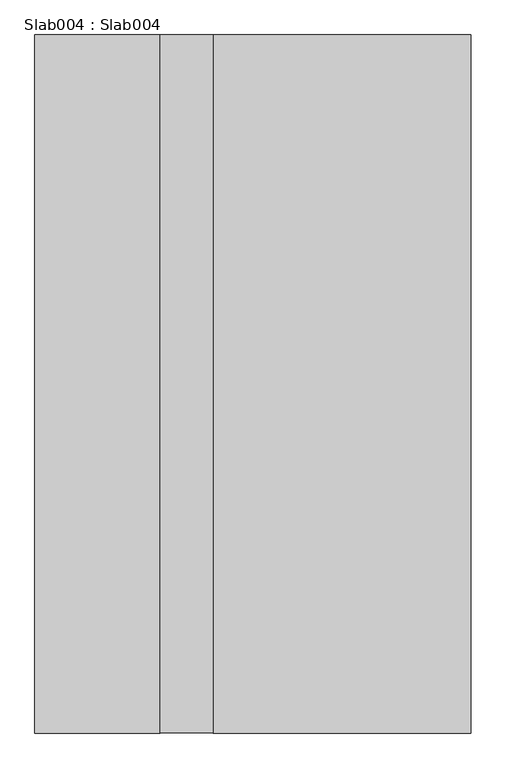
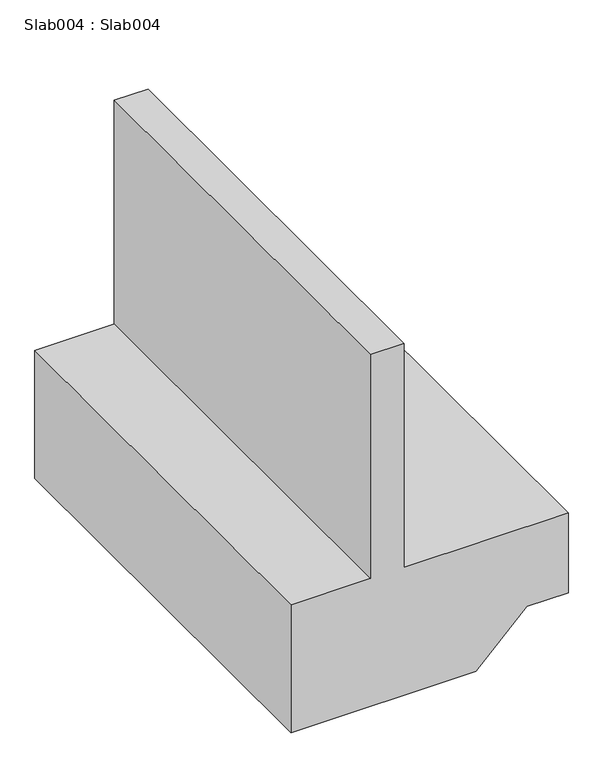
"""IFC4 building model written with IfcOpenShell, lengths in millimetres: proxy geometry, Slab004 : Slab004."""

from ifc_helpers import new_model, si_unit, frame, origin, place, context, project, spatial, polyline, outline, extrude, source, transform, mapped, element, save


def slab004_slab004_fb29ce74(model_context):
    return source(origin(), model_context, "Body", "SweptSolid", [
        extrude(outline(polyline([(32568.8960253, -9507.921316), (33635.6960253, -9507.921316), (33635.6960253, -9660.321316), (32568.8960253, -9660.321316), (32568.8960253, -10018.8790435), (31959.2960253, -10018.8790435), (31959.2960253, -9184.0737014), (32187.8960253, -8955.4737014), (32187.8960253, -8768.5299994), (32568.8960253, -8768.5299994), (32568.8960253, -9507.921316)])), frame((0.0, 7182.1529359, 0.0), z_axis=(0.0, 1.0, 0.0), x_axis=(0.0, 0.0, 1.0)), (0.0, 0.0, 1.0), 2000.0),
    ])


if __name__ == "__main__":
    model = new_model("IFC4")
    model_context = context("Model", 3, world=origin())
    ifc_project = project(units=[si_unit("LENGTHUNIT", "METRE", prefix="MILLI")], contexts=[model_context])
    site = spatial("IfcSite", under=ifc_project)
    building = spatial("IfcBuilding", under=site)
    placement = place(None, origin())
    slab004_slab004_shape = slab004_slab004_fb29ce74(model_context)
    element("IfcBuildingElementProxy", 1, Name="Slab004 : Slab004", ObjectType="Slab004 : Slab004", at=placement, inside=building, context=model_context, shape_type="MappedRepresentation", body=[
        mapped(slab004_slab004_shape, transform((0.0, 0.0, 0.0), x_axis=(1.0, 0.0, 0.0), y_axis=(0.0, 1.0, 0.0), z_axis=(0.0, 0.0, 1.0))),
    ])
    save(model, "model.ifc")

# Revit data of these elements
# Type "Slab004 : Slab004"
#   NameOverride = "Slab004"
# Element 1 (IfcBuildingElementProxy, "Slab004 : Slab004")
#   Materials on its faces: "CONCRETE SLAB W/ GRADE BEAM (SEE STRUCT DWGS)"
# Materials
#   "CONCRETE SLAB W/ GRADE BEAM (SEE STRUCT DWGS)": class "Unassigned", colour RGB 128 128 128, transparency 0, Cost = 0
